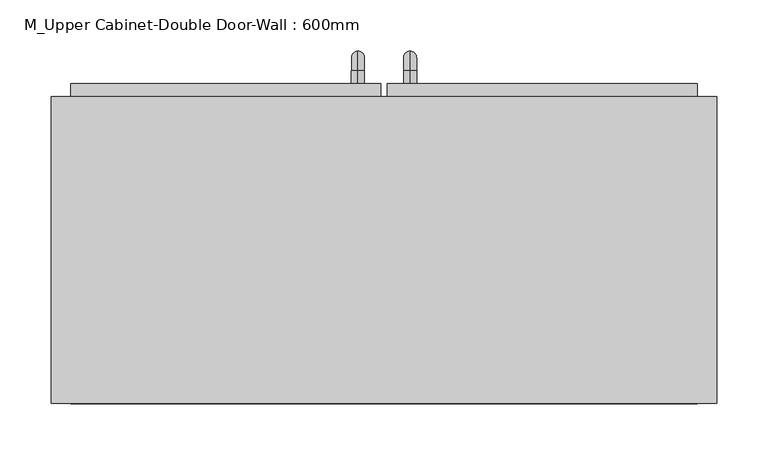
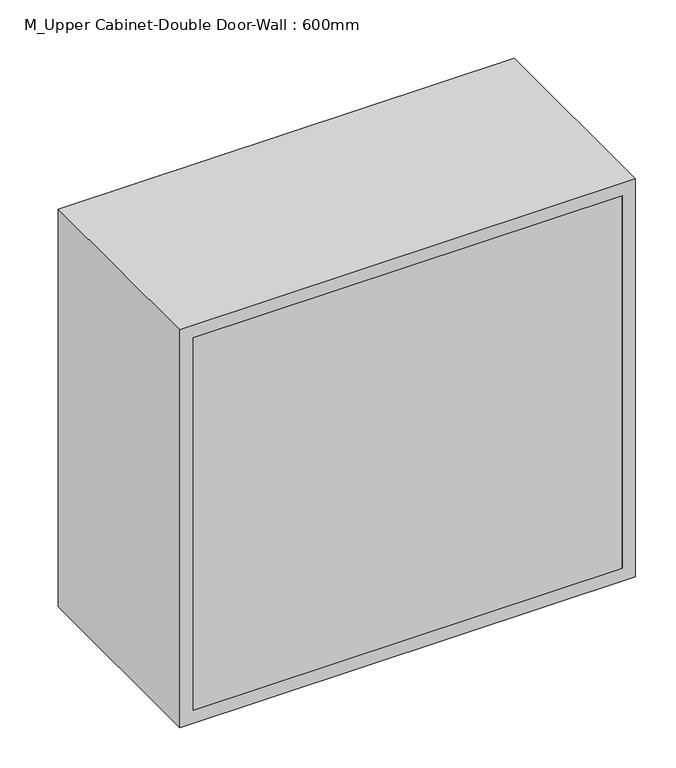
"""IFC4 building model written with IfcOpenShell, lengths in millimetres: furniture geometry, M_Upper Cabinet-Double Door-Wall : 600mm."""

from ifc_helpers import new_model, si_unit, point, frame, origin, place, context, project, spatial, polyline, circle_curve, ellipse_curve, trimmed, outline, extrude, source, transform, mapped, element, save
from ifc_brep_helpers import plane_surface, cylinder_surface, revolved_surface, advanced_brep


def m_upper_cabinet_double_door_wall_600mm_a5d0a472(model_context):
    return source(origin(), model_context, "Body", "SolidModel", [
        advanced_brep(
        [(55.1711628, 387.7, 1546.05), (55.1711628, 387.7, 1558.75), (55.1711628, 400.4, 1546.05), (55.1711628, 400.4, 1558.75), (55.1711628, 419.45, 1539.7), (55.1711628, 406.75, 1539.7), (55.1711628, 406.75, 1463.5), (55.1711628, 419.45, 1463.5), (55.1711628, 400.4, 1444.45), (55.1711628, 400.4, 1457.15), (55.1711628, 387.7, 1457.15), (55.1711628, 387.7, 1444.45)],
        [
            (0, 1, circle_curve(frame((55.1711628, 387.7, 1552.4), z_axis=(0.0, -1.0, 0.0), x_axis=(0.0, 0.0, -1.0)), 6.35)),
            (1, 0, circle_curve(frame((55.1711628, 387.7, 1552.4), z_axis=(0.0, -1.0, 0.0), x_axis=(0.0, 0.0, -1.0)), 6.35)),
            (0, 2),
            (2, 3, circle_curve(frame((55.1711628, 400.4, 1552.4), z_axis=(0.0, -1.0, 0.0), x_axis=(0.0, 0.0, -1.0)), 6.35)),
            (3, 1),
            (3, 2, circle_curve(frame((55.1711628, 400.4, 1552.4), z_axis=(0.0, -1.0, 0.0), x_axis=(0.0, 0.0, -1.0)), 6.35)),
            (4, 3, circle_curve(frame((55.1711628, 400.4, 1539.7), z_axis=(1.0, 0.0, 0.0), x_axis=(0.0, 0.0, 1.0)), 19.05)),
            (2, 5, circle_curve(frame((55.1711628, 400.4, 1539.7), z_axis=(-1.0, 0.0, 0.0), x_axis=(0.0, 0.0, 1.0)), 6.35)),
            (5, 4, circle_curve(frame((55.1711628, 413.1, 1539.7), z_axis=(0.0, 0.0, 1.0), x_axis=(0.0, -1.0, 0.0)), 6.35)),
            (4, 5, circle_curve(frame((55.1711628, 413.1, 1539.7), z_axis=(0.0, 0.0, 1.0), x_axis=(0.0, -1.0, 0.0)), 6.35)),
            (5, 6),
            (6, 7, circle_curve(frame((55.1711628, 413.1, 1463.5), z_axis=(0.0, 0.0, 1.0), x_axis=(0.0, -1.0, 0.0)), 6.35)),
            (7, 4),
            (7, 6, circle_curve(frame((55.1711628, 413.1, 1463.5), z_axis=(0.0, 0.0, 1.0), x_axis=(0.0, -1.0, 0.0)), 6.35)),
            (8, 7, circle_curve(frame((55.1711628, 400.4, 1463.5), z_axis=(1.0, 0.0, 0.0), x_axis=(0.0, 1.0, 0.0)), 19.05)),
            (6, 9, circle_curve(frame((55.1711628, 400.4, 1463.5), z_axis=(-1.0, 0.0, 0.0), x_axis=(0.0, 1.0, 0.0)), 6.35)),
            (9, 8, circle_curve(frame((55.1711628, 400.4, 1450.8), z_axis=(0.0, 1.0, 0.0), x_axis=(0.0, 0.0, 1.0)), 6.35)),
            (8, 9, circle_curve(frame((55.1711628, 400.4, 1450.8), z_axis=(0.0, 1.0, 0.0), x_axis=(0.0, 0.0, 1.0)), 6.35)),
            (10, 11, circle_curve(frame((55.1711628, 387.7, 1450.8), z_axis=(0.0, -1.0, 0.0), x_axis=(0.0, 0.0, 1.0)), 6.35)),
            (11, 10, circle_curve(frame((55.1711628, 387.7, 1450.8), z_axis=(0.0, -1.0, 0.0), x_axis=(0.0, 0.0, 1.0)), 6.35)),
            (9, 10),
            (11, 8),
        ],
        [
            plane_surface(frame((48.8211628, 387.7, 1552.4), z_axis=(0.0, -1.0, 0.0), x_axis=(0.0, 0.0, 1.0))),
            cylinder_surface(frame((55.1711628, 387.7, 1552.4), z_axis=(0.0, -1.0, 0.0), x_axis=(0.0, 0.0, -1.0)), 6.35),
            revolved_surface(trimmed(ellipse_curve(frame((55.1711628, 400.4, 1552.4), z_axis=(0.0, -1.0, 0.0), x_axis=(0.0, 0.0, -1.0)), 6.35, 6.35), [point((55.1711628, 400.4, 1546.05))], [point((55.1711628, 400.4, 1558.75))], True, "CARTESIAN"), (55.1711628, 400.4, 1539.7), (-1.0, 0.0, 0.0)),
            revolved_surface(trimmed(ellipse_curve(frame((55.1711628, 400.4, 1552.4), z_axis=(0.0, -1.0, 0.0), x_axis=(0.0, 0.0, -1.0)), 6.35, 6.35), [point((55.1711628, 400.4, 1558.75))], [point((55.1711628, 400.4, 1546.05))], True, "CARTESIAN"), (55.1711628, 400.4, 1539.7), (-1.0, 0.0, 0.0)),
            cylinder_surface(frame((55.1711628, 413.1, 1539.7), z_axis=(0.0, 0.0, 1.0), x_axis=(0.0, -1.0, 0.0)), 6.35),
            revolved_surface(trimmed(ellipse_curve(frame((55.1711628, 413.1, 1463.5), z_axis=(0.0, 0.0, 1.0), x_axis=(0.0, -1.0, 0.0)), 6.35, 6.35), [point((55.1711628, 406.75, 1463.5))], [point((55.1711628, 419.45, 1463.5))], True, "CARTESIAN"), (55.1711628, 400.4, 1463.5), (-1.0, 0.0, 0.0)),
            revolved_surface(trimmed(ellipse_curve(frame((55.1711628, 413.1, 1463.5), z_axis=(0.0, 0.0, 1.0), x_axis=(0.0, -1.0, 0.0)), 6.35, 6.35), [point((55.1711628, 419.45, 1463.5))], [point((55.1711628, 406.75, 1463.5))], True, "CARTESIAN"), (55.1711628, 400.4, 1463.5), (-1.0, 0.0, 0.0)),
            plane_surface(frame((48.8211628, 387.7, 1450.8), z_axis=(0.0, -1.0, 0.0), x_axis=(0.0, 0.0, -1.0))),
            cylinder_surface(frame((55.1711628, 400.4, 1450.8), z_axis=(0.0, 1.0, 0.0), x_axis=(0.0, 0.0, 1.0)), 6.35),
        ],
        [
            (0, [[1, 2]]),
            (1, [[-1, 3, 4, 5]]),
            (1, [[-2, -5, 6, -3]]),
            (2, [[7, -4, 8, 9]]),
            (3, [[-8, -6, -7, 10]]),
            (4, [[-9, 11, 12, 13]]),
            (4, [[-10, -13, 14, -11]]),
            (5, [[15, -12, 16, 17]]),
            (6, [[-16, -14, -15, 18]]),
            (7, [[19, 20]]),
            (8, [[-17, 21, -20, 22]]),
            (8, [[-18, -22, -19, -21]]),
        ],
    ),
        advanced_brep(
        [(4.3711628, 387.7, 1546.05), (4.3711628, 387.7, 1558.75), (4.3711628, 400.4, 1546.05), (4.3711628, 400.4, 1558.75), (4.3711628, 419.45, 1539.7), (4.3711628, 406.75, 1539.7), (4.3711628, 406.75, 1463.5), (4.3711628, 419.45, 1463.5), (4.3711628, 400.4, 1444.45), (4.3711628, 400.4, 1457.15), (4.3711628, 387.7, 1457.15), (4.3711628, 387.7, 1444.45)],
        [
            (0, 1, circle_curve(frame((4.3711628, 387.7, 1552.4), z_axis=(0.0, -1.0, 0.0), x_axis=(0.0, 0.0, 1.0)), 6.35)),
            (1, 0, circle_curve(frame((4.3711628, 387.7, 1552.4), z_axis=(0.0, -1.0, 0.0), x_axis=(0.0, 0.0, 1.0)), 6.35)),
            (0, 2),
            (2, 3, circle_curve(frame((4.3711628, 400.4, 1552.4), z_axis=(0.0, -1.0, 0.0), x_axis=(0.0, 0.0, 1.0)), 6.35)),
            (3, 1),
            (3, 2, circle_curve(frame((4.3711628, 400.4, 1552.4), z_axis=(0.0, -1.0, 0.0), x_axis=(0.0, 0.0, 1.0)), 6.35)),
            (4, 3, circle_curve(frame((4.3711628, 400.4, 1539.7), z_axis=(1.0, 0.0, 0.0), x_axis=(0.0, 0.0, 1.0)), 19.05)),
            (2, 5, circle_curve(frame((4.3711628, 400.4, 1539.7), z_axis=(-1.0, 0.0, 0.0), x_axis=(0.0, 0.0, 1.0)), 6.35)),
            (5, 4, circle_curve(frame((4.3711628, 413.1, 1539.7), z_axis=(0.0, 0.0, 1.0), x_axis=(0.0, 1.0, 0.0)), 6.35)),
            (4, 5, circle_curve(frame((4.3711628, 413.1, 1539.7), z_axis=(0.0, 0.0, 1.0), x_axis=(0.0, 1.0, 0.0)), 6.35)),
            (5, 6),
            (6, 7, circle_curve(frame((4.3711628, 413.1, 1463.5), z_axis=(0.0, 0.0, 1.0), x_axis=(0.0, 1.0, 0.0)), 6.35)),
            (7, 4),
            (7, 6, circle_curve(frame((4.3711628, 413.1, 1463.5), z_axis=(0.0, 0.0, 1.0), x_axis=(0.0, 1.0, 0.0)), 6.35)),
            (8, 7, circle_curve(frame((4.3711628, 400.4, 1463.5), z_axis=(1.0, 0.0, 0.0), x_axis=(0.0, 1.0, 0.0)), 19.05)),
            (6, 9, circle_curve(frame((4.3711628, 400.4, 1463.5), z_axis=(-1.0, 0.0, 0.0), x_axis=(0.0, 1.0, 0.0)), 6.35)),
            (9, 8, circle_curve(frame((4.3711628, 400.4, 1450.8), z_axis=(0.0, 1.0, 0.0), x_axis=(0.0, 0.0, -1.0)), 6.35)),
            (8, 9, circle_curve(frame((4.3711628, 400.4, 1450.8), z_axis=(0.0, 1.0, 0.0), x_axis=(0.0, 0.0, -1.0)), 6.35)),
            (10, 11, circle_curve(frame((4.3711628, 387.7, 1450.8), z_axis=(0.0, -1.0, 0.0), x_axis=(0.0, 0.0, -1.0)), 6.35)),
            (11, 10, circle_curve(frame((4.3711628, 387.7, 1450.8), z_axis=(0.0, -1.0, 0.0), x_axis=(0.0, 0.0, -1.0)), 6.35)),
            (9, 10),
            (11, 8),
        ],
        [
            plane_surface(frame((-1.9788372, 387.7, 1552.4), z_axis=(0.0, -1.0, 0.0), x_axis=(0.0, 0.0, 1.0))),
            cylinder_surface(frame((4.3711628, 387.7, 1552.4), z_axis=(0.0, -1.0, 0.0), x_axis=(0.0, 0.0, 1.0)), 6.35),
            revolved_surface(trimmed(ellipse_curve(frame((4.3711628, 400.4, 1552.4), z_axis=(0.0, -1.0, 0.0), x_axis=(0.0, 0.0, 1.0)), 6.35, 6.35), [point((4.3711628, 400.4, 1546.05))], [point((4.3711628, 400.4, 1558.75))], True, "CARTESIAN"), (4.3711628, 400.4, 1539.7), (-1.0, 0.0, 0.0)),
            revolved_surface(trimmed(ellipse_curve(frame((4.3711628, 400.4, 1552.4), z_axis=(0.0, -1.0, 0.0), x_axis=(0.0, 0.0, 1.0)), 6.35, 6.35), [point((4.3711628, 400.4, 1558.75))], [point((4.3711628, 400.4, 1546.05))], True, "CARTESIAN"), (4.3711628, 400.4, 1539.7), (-1.0, 0.0, 0.0)),
            cylinder_surface(frame((4.3711628, 413.1, 1539.7), z_axis=(0.0, 0.0, 1.0), x_axis=(0.0, 1.0, 0.0)), 6.35),
            revolved_surface(trimmed(ellipse_curve(frame((4.3711628, 413.1, 1463.5), z_axis=(0.0, 0.0, 1.0), x_axis=(0.0, 1.0, 0.0)), 6.35, 6.35), [point((4.3711628, 406.75, 1463.5))], [point((4.3711628, 419.45, 1463.5))], True, "CARTESIAN"), (4.3711628, 400.4, 1463.5), (-1.0, 0.0, 0.0)),
            revolved_surface(trimmed(ellipse_curve(frame((4.3711628, 413.1, 1463.5), z_axis=(0.0, 0.0, 1.0), x_axis=(0.0, 1.0, 0.0)), 6.35, 6.35), [point((4.3711628, 419.45, 1463.5))], [point((4.3711628, 406.75, 1463.5))], True, "CARTESIAN"), (4.3711628, 400.4, 1463.5), (-1.0, 0.0, 0.0)),
            plane_surface(frame((-1.9788372, 387.7, 1450.8), z_axis=(0.0, -1.0, 0.0), x_axis=(0.0, 0.0, -1.0))),
            cylinder_surface(frame((4.3711628, 400.4, 1450.8), z_axis=(0.0, 1.0, 0.0), x_axis=(0.0, 0.0, -1.0)), 6.35),
        ],
        [
            (0, [[1, 2]]),
            (1, [[-1, 3, 4, 5]]),
            (1, [[-2, -5, 6, -3]]),
            (2, [[7, -4, 8, 9]]),
            (3, [[-8, -6, -7, 10]]),
            (4, [[-9, 11, 12, 13]]),
            (4, [[-10, -13, 14, -11]]),
            (5, [[15, -12, 16, 17]]),
            (6, [[-16, -14, -15, 18]]),
            (7, [[19, 20]]),
            (8, [[-17, 21, -20, 22]]),
            (8, [[-18, -22, -19, -21]]),
        ],
    ),
        extrude(outline(polyline([(32.9461628, 387.7), (335.7211628, 387.7), (335.7211628, 355.95), (32.9461628, 355.95), (32.9461628, 387.7)])), frame((0.0, 0.0, 1419.05), z_axis=(0.0, 0.0, 1.0), x_axis=(1.0, 0.0, 0.0)), (0.0, 0.0, 1.0), 561.9),
        extrude(outline(polyline([(-276.1788372, 387.7), (26.5961628, 387.7), (26.5961628, 355.95), (-276.1788372, 355.95), (-276.1788372, 387.7)])), frame((0.0, 0.0, 1419.05), z_axis=(0.0, 0.0, 1.0), x_axis=(1.0, 0.0, 0.0)), (0.0, 0.0, 1.0), 561.9),
        extrude(outline(polyline([(335.7211628, 75.0), (-276.1788372, 75.0), (-276.1788372, 94.05), (335.7211628, 94.05), (335.7211628, 75.0)])), frame((0.0, 0.0, 1419.05), z_axis=(0.0, 0.0, 1.0), x_axis=(1.0, 0.0, 0.0)), (0.0, 0.0, 1.0), 561.9),
        extrude(outline(polyline([(2000.0, -295.2288372), (1400.0, -295.2288372), (1400.0, 354.7711628), (2000.0, 354.7711628), (2000.0, -295.2288372)]), holes=[polyline([(1980.95, -276.1788372), (1980.95, 335.7211628), (1419.05, 335.7211628), (1419.05, -276.1788372), (1980.95, -276.1788372)])]), frame((0.0, 75.0, 0.0), z_axis=(0.0, 1.0, 0.0), x_axis=(0.0, 0.0, 1.0)), (0.0, 0.0, 1.0), 300.0),
    ])


if __name__ == "__main__":
    model = new_model("IFC4")
    model_context = context("Model", 3, world=origin())
    ifc_project = project(units=[si_unit("LENGTHUNIT", "METRE", prefix="MILLI")], contexts=[model_context])
    site = spatial("IfcSite", under=ifc_project)
    building = spatial("IfcBuilding", under=site)
    placement = place(None, origin())
    m_upper_cabinet_double_door_wall_600mm_shape = m_upper_cabinet_double_door_wall_600mm_a5d0a472(model_context)
    element("IfcFurniture", 1, ObjectType="M_Upper Cabinet-Double Door-Wall : 600mm", at=placement, inside=building, context=model_context, shape_type="MappedRepresentation", body=[
        mapped(m_upper_cabinet_double_door_wall_600mm_shape, transform((0.0, 0.0, 0.0), x_axis=(1.0, 0.0, 0.0), y_axis=(0.0, 1.0, 0.0), z_axis=(0.0, 0.0, 1.0))),
    ])
    save(model, "model.ifc")

# Revit data of these elements
# Type "M_Upper Cabinet-Double Door-Wall : 600mm"
#   Depth = 0.3 m
#   Height = 0.6 m
#   Top Of Cabinet = 2 m
#   Width = 0.65 m
#   Cabinet Material = book white
#   Door/Drawer Material = none
#   Handle Material = Cabinets - Handles
#   Default Elevation = 0
# Element 1 (IfcFurniture, "M_Upper Cabinet-Double Door-Wall : 600mm")
#   Materials on its faces: "Cabinets - Handles", "book white", "Cabinets"
# Materials
#   "book white": class "Paint", colour RGB 211 193 153, transparency 0
#   "Cabinets - Handles": class "Metal", colour RGB 57 57 57, transparency 0
#   "Cabinets": class "Miscellaneous", colour RGB 249 249 249, transparency 0
